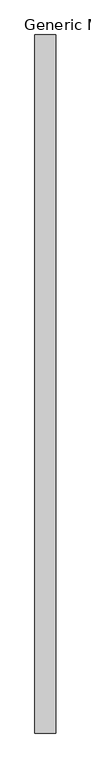
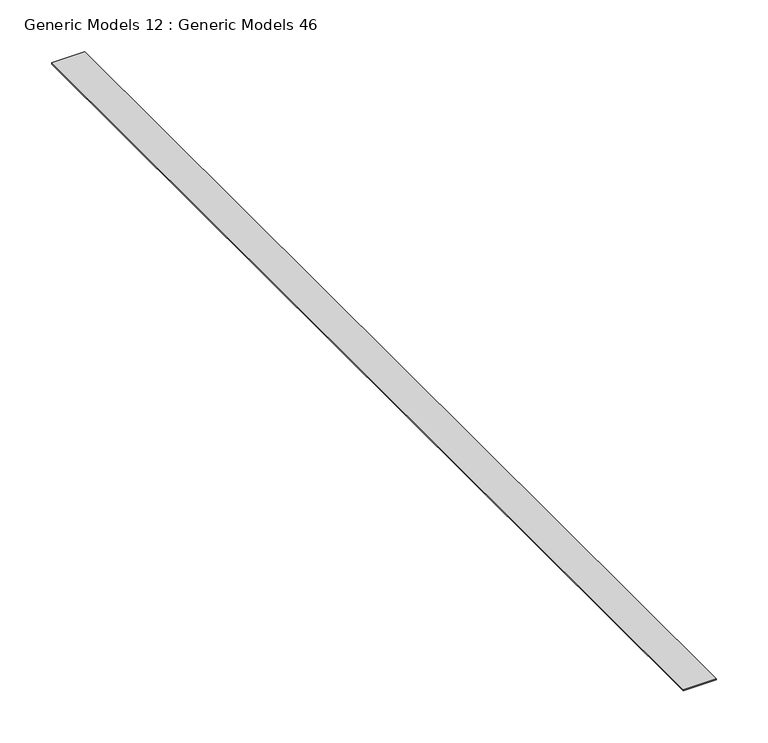
"""IFC4 building model written with IfcOpenShell, lengths in millimetres: proxy geometry, Generic Models 12 : Generic Models 46."""

import ifcopenshell
import ifcopenshell.guid

model = None  # the IFC model being written
_history = None  # IfcOwnerHistory: only IFC2X3 demands one
_inside = {}  # id of a spatial element -> (the spatial element, [elements in it])
_under = {}  # id of a project, library or spatial element -> (it, [spatial elements below it])
_declared = {}  # id of a project -> (the project, [libraries it declares])
_typed = {}  # id of a type object -> (the type object, [elements of that type])
_made_of = {}  # id of a material, layer set ... -> (it, [elements and type objects made of it])


def new_model(schema):
    """Start an empty IFC model of exactly this schema.

    Asked for "IFC4X3", IfcOpenShell would pick the latest addendum, in which some entities
    have other attributes; the version numbers below select the first issue.
    IFC2X3 requires an IfcOwnerHistory on every rooted entity: one is made here for all.
    """
    global model, _history
    if schema == "IFC4X3":
        model = ifcopenshell.file(schema_version=(4, 3, 0, 0))
    else:
        model = ifcopenshell.file(schema=schema)
    _inside.clear()
    _under.clear()
    _declared.clear()
    _typed.clear()
    _made_of.clear()
    _history = None
    if model.schema == "IFC2X3":
        org = make("IfcOrganization", Name="unknown")
        user = make(
            "IfcPersonAndOrganization",
            ThePerson=make("IfcPerson", FamilyName="unknown"),
            TheOrganization=org,
        )
        app = make(
            "IfcApplication",
            ApplicationDeveloper=org,
            Version="unknown",
            ApplicationFullName="unknown",
            ApplicationIdentifier="unknown",
        )
        _history = make(
            "IfcOwnerHistory",
            OwningUser=user,
            OwningApplication=app,
            ChangeAction="ADDED",
            CreationDate=0,
        )
    return model


def make(cls, **values):
    """One entity of the class cls with the attributes given. An attribute that is None is left unset."""
    return model.create_entity(
        cls, **{name: value for name, value in values.items() if value is not None}
    )


def rooted(cls, **values):
    """An entity with a GlobalId (a new one), such as an element, a storey or a relation."""
    return make(cls, GlobalId=ifcopenshell.guid.new(), OwnerHistory=_history, **values)


def si_unit(unit_type, name, prefix=None):
    """IfcSIUnit, for example si_unit("LENGTHUNIT", "METRE", prefix="MILLI")."""
    return make("IfcSIUnit", UnitType=unit_type, Prefix=prefix, Name=name)


def assignment(units):
    """IfcUnitAssignment: the units of a project."""
    return None if units is None else make("IfcUnitAssignment", Units=units)


def point(xyz):
    """IfcCartesianPoint."""
    return None if xyz is None else make("IfcCartesianPoint", Coordinates=xyz)


def direction(xyz):
    """IfcDirection."""
    return None if xyz is None else make("IfcDirection", DirectionRatios=xyz)


def frame(location, z_axis=None, x_axis=None):
    """IfcAxis2Placement3D, a coordinate frame: its origin and axes. An axis left out is left unset."""
    return make(
        "IfcAxis2Placement3D",
        Location=point(location),
        Axis=direction(z_axis),
        RefDirection=direction(x_axis),
    )


def origin():
    """The frame at (0, 0, 0) with its axes left unset."""
    return frame((0.0, 0.0, 0.0))


def place(relative_to, where):
    """IfcLocalPlacement: puts the frame where relative to a parent placement (None: the world)."""
    return make(
        "IfcLocalPlacement", PlacementRelTo=relative_to, RelativePlacement=where
    )


def context(
    kind, dimensions, precision=None, world=None, true_north=None, identifier=None
):
    """IfcGeometricRepresentationContext, for example the 3D "Model" context."""
    return make(
        "IfcGeometricRepresentationContext",
        ContextIdentifier=identifier,
        ContextType=kind,
        CoordinateSpaceDimension=dimensions,
        Precision=precision,
        WorldCoordinateSystem=world,
        TrueNorth=true_north,
    )


def project(units=None, contexts=None):
    """IfcProject with its units and contexts."""
    return rooted(
        "IfcProject",
        Name="project",
        RepresentationContexts=contexts,
        UnitsInContext=assignment(units),
    )


def spatial(cls, under=None, at=None, **own):
    """A site, building, storey or space (cls), placed at a placement, below another one or the project."""
    s = rooted(cls, ObjectPlacement=at, **own)
    if under is not None:
        _under.setdefault(under.id(), (under, []))[1].append(s)
    return s


def polyline(points):
    """IfcPolyline through the points."""
    return make("IfcPolyline", Points=[point(p) for p in points])


def outline(outer, holes=None, kind="AREA"):
    """IfcArbitraryClosedProfileDef: a profile drawn as a closed curve; with holes, ...WithVoids."""
    if holes is None:
        return make("IfcArbitraryClosedProfileDef", ProfileType=kind, OuterCurve=outer)
    return make(
        "IfcArbitraryProfileDefWithVoids",
        ProfileType=kind,
        OuterCurve=outer,
        InnerCurves=holes,
    )


def extrude(swept, where, along, depth):
    """IfcExtrudedAreaSolid: the profile swept, set in the frame where, extruded along a direction by depth."""
    return make(
        "IfcExtrudedAreaSolid",
        SweptArea=swept,
        Position=where,
        ExtrudedDirection=direction(along),
        Depth=depth,
    )


def shape(context_of_items, identifier, shape_type, items):
    """IfcShapeRepresentation: the items that make up one representation, for example the "Body"."""
    return make(
        "IfcShapeRepresentation",
        ContextOfItems=context_of_items,
        RepresentationIdentifier=identifier,
        RepresentationType=shape_type,
        Items=items,
    )


def source(mapping_origin, context_of_items, identifier, shape_type, items):
    """IfcRepresentationMap: a shape defined once, which mapped items show again and again."""
    return make(
        "IfcRepresentationMap",
        MappingOrigin=mapping_origin,
        MappedRepresentation=shape(context_of_items, identifier, shape_type, items),
    )


def transform(
    local_origin,
    x_axis=None,
    y_axis=None,
    z_axis=None,
    scale=None,
    scale2=None,
    scale3=None,
    uniform=True,
):
    """IfcCartesianTransformationOperator3D, or its non-uniform kind. x_axis, y_axis, z_axis: its Axis1, 2, 3."""
    if uniform:
        return make(
            "IfcCartesianTransformationOperator3D",
            Axis1=direction(x_axis),
            Axis2=direction(y_axis),
            LocalOrigin=point(local_origin),
            Scale=scale,
            Axis3=direction(z_axis),
        )
    return make(
        "IfcCartesianTransformationOperator3DnonUniform",
        Axis1=direction(x_axis),
        Axis2=direction(y_axis),
        LocalOrigin=point(local_origin),
        Scale=scale,
        Axis3=direction(z_axis),
        Scale2=scale2,
        Scale3=scale3,
    )


def mapped(mapping_source, mapping_target):
    """IfcMappedItem: shows the shape of a source again, moved by a transform."""
    return make(
        "IfcMappedItem", MappingSource=mapping_source, MappingTarget=mapping_target
    )


def made_of(thing, what):
    """Note that an element or type object is made of a material, layer set ...; save() writes the relation."""
    if what is not None:
        _made_of.setdefault(what.id(), (what, []))[1].append(thing)
    return thing


def element(
    cls,
    number,
    at=None,
    inside=None,
    cuts=None,
    type_object=None,
    material=None,
    context=None,
    identifier="Body",
    shape_type=None,
    held_by="IfcProductDefinitionShape",
    body=None,
    shapes=None,
    **own,
):
    """One element of the class cls, such as IfcWall. Its Tag is "e" and its number.

    at: its placement. inside: the storey or other place that contains it. cuts: it is an
    opening in that element (IfcRelVoidsElement). A single representation is given by context,
    identifier, shape_type and body (its items); several are given by shapes. held_by: the class
    of the entity that holds the representations. save() writes the other relations.
    """
    e = rooted(cls, Tag="e%d" % number, ObjectPlacement=at, **own)
    if body is not None:
        shapes = [shape(context, identifier, shape_type, body)]
    if shapes is not None:
        e.Representation = make(held_by, Representations=shapes)
    if inside is not None:
        _inside.setdefault(inside.id(), (inside, []))[1].append(e)
    if cuts is not None:
        rooted(
            "IfcRelVoidsElement", RelatingBuildingElement=cuts, RelatedOpeningElement=e
        )
    if type_object is not None:
        _typed.setdefault(type_object.id(), (type_object, []))[1].append(e)
    return made_of(e, material)


def aggregate(whole, parts):
    """IfcRelAggregates: a whole, such as a stair, and the parts it consists of."""
    return rooted("IfcRelAggregates", RelatingObject=whole, RelatedObjects=parts)


def save(model, path):
    """Write the relations noted so far, then the file.

    IfcRelAggregates (storeys below a building ...), IfcRelContainedInSpatialStructure (elements
    in a storey), IfcRelDefinesByType, IfcRelAssociatesMaterial and IfcRelDeclares: one each for
    every whole, place, type object, material and project.
    """
    for whole, parts in _under.values():
        aggregate(whole, parts)
    for where, things in _inside.values():
        rooted(
            "IfcRelContainedInSpatialStructure",
            RelatedElements=things,
            RelatingStructure=where,
        )
    for kind, things in _typed.values():
        rooted("IfcRelDefinesByType", RelatedObjects=things, RelatingType=kind)
    for what, things in _made_of.values():
        rooted("IfcRelAssociatesMaterial", RelatedObjects=things, RelatingMaterial=what)
    for by, libraries in _declared.values():
        rooted("IfcRelDeclares", RelatingContext=by, RelatedDefinitions=libraries)
    model.write(path)


def generic_models_12_generic_models_46_b8a9a4e8(model_context):
    return source(origin(), model_context, "Body", "SweptSolid", [
        extrude(outline(polyline([(49757.8505137, 0.0), (49721.1284797, 0.0), (49721.1284797, 1219.2), (49757.8505137, 1219.2), (49757.8505137, 0.0)])), frame((0.0, 0.0, 5505.7509163), z_axis=(0.0, 0.0, 1.0), x_axis=(1.0, 0.0, 0.0)), (0.0, 0.0, 1.0), 1.5875),
    ])


if __name__ == "__main__":
    model = new_model("IFC4")
    model_context = context("Model", 3, world=origin())
    ifc_project = project(units=[si_unit("LENGTHUNIT", "METRE", prefix="MILLI")], contexts=[model_context])
    site = spatial("IfcSite", under=ifc_project)
    building = spatial("IfcBuilding", under=site)
    placement = place(None, origin())
    generic_models_12_generic_models_46_shape = generic_models_12_generic_models_46_b8a9a4e8(model_context)
    element("IfcBuildingElementProxy", 1, Name="Generic Models 12 : Generic Models 46", ObjectType="Generic Models 12 : Generic Models 46", at=placement, inside=building, context=model_context, shape_type="MappedRepresentation", body=[
        mapped(generic_models_12_generic_models_46_shape, transform((0.0, 0.0, 0.0), x_axis=(1.0, 0.0, 0.0), y_axis=(0.0, 1.0, 0.0), z_axis=(0.0, 0.0, 1.0))),
    ])
    save(model, "model.ifc")

# Revit data of these elements
# Element 1 (IfcBuildingElementProxy, "Generic Models 12 : Generic Models 46")
#   Materials on its faces: "SET IN BED OF SEALANT"
# Materials
#   "SET IN BED OF SEALANT": class "Unassigned", colour RGB 58 208 21, transparency 0, Cost = 0
